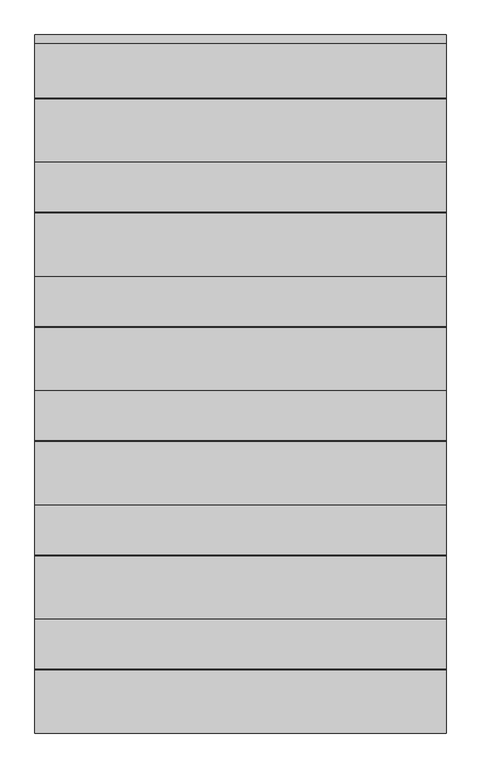
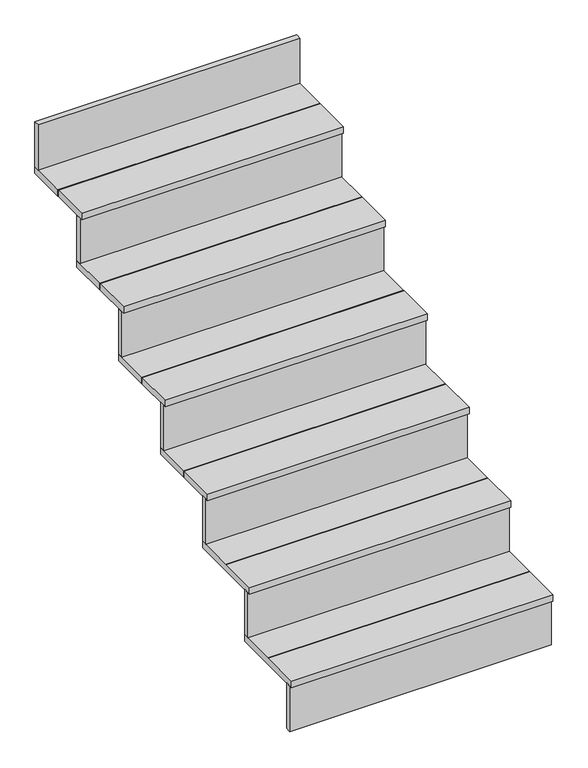
"""IFC4 building model written with IfcOpenShell, lengths in millimetres: stair flight geometry."""

from ifc_helpers import new_model, si_unit, frame, origin, origin_with_axes, place, context, project, spatial, polyline, outline, extrude, source, transform, mapped, element, save


def stair_flight_64412767(model_context):
    return source(origin(), model_context, "Body", "SweptSolid", [
        extrude(outline(polyline([(-21667.4414763, -10959.3570712), (-21667.4414763, -10978.4070712), (-22581.8414763, -10978.4070712), (-22581.8414763, -10959.3570712), (-21667.4414763, -10959.3570712)])), origin_with_axes(), (0.0, 0.0, 1.0), 167.8582813),
        extrude(outline(polyline([(-10848.2320712, 167.8582812), (-10987.9320712, 167.8582812), (-10987.9320712, 191.77), (-10848.2320712, 191.77), (-10848.2320712, 180.0157279), (-10845.0570712, 180.0157279), (-10845.0570712, 191.77), (-10705.3570712, 191.77), (-10705.3570712, 167.8582812), (-10845.0570712, 167.8582812), (-10845.0570712, 179.6125533), (-10848.2320712, 179.6125533), (-10848.2320712, 167.8582812)])), frame((-22581.8414763, 0.0, 0.0), z_axis=(1.0, 0.0, 0.0), x_axis=(0.0, 1.0, 0.0)), (0.0, 0.0, 1.0), 914.4),
        extrude(outline(polyline([(-21667.4414763, -10705.3570712), (-21667.4414763, -10724.4070712), (-22581.8414763, -10724.4070712), (-22581.8414763, -10705.3570712), (-21667.4414763, -10705.3570712)])), frame((0.0, 0.0, 191.77), z_axis=(0.0, 0.0, 1.0), x_axis=(1.0, 0.0, 0.0)), (0.0, 0.0, 1.0), 167.8582813),
        extrude(outline(polyline([(-10594.2320712, 359.6282812), (-10733.9320712, 359.6282812), (-10733.9320712, 383.54), (-10594.2320712, 383.54), (-10594.2320712, 371.7857279), (-10591.0570712, 371.7857279), (-10591.0570712, 383.54), (-10451.3570712, 383.54), (-10451.3570712, 359.6282812), (-10591.0570712, 359.6282812), (-10591.0570712, 371.3825533), (-10594.2320712, 371.3825533), (-10594.2320712, 359.6282812)])), frame((-22581.8414763, 0.0, 0.0), z_axis=(1.0, 0.0, 0.0), x_axis=(0.0, 1.0, 0.0)), (0.0, 0.0, 1.0), 914.4),
        extrude(outline(polyline([(-21667.4414763, -10451.3570712), (-21667.4414763, -10470.4070712), (-22581.8414763, -10470.4070712), (-22581.8414763, -10451.3570712), (-21667.4414763, -10451.3570712)])), frame((0.0, 0.0, 383.54), z_axis=(0.0, 0.0, 1.0), x_axis=(1.0, 0.0, 0.0)), (0.0, 0.0, 1.0), 167.8582813),
        extrude(outline(polyline([(-10340.2320712, 551.3982812), (-10479.9320712, 551.3982812), (-10479.9320712, 575.31), (-10340.2320712, 575.31), (-10340.2320712, 563.5557279), (-10337.0570712, 563.5557279), (-10337.0570712, 575.31), (-10197.3570712, 575.31), (-10197.3570712, 551.3982812), (-10337.0570712, 551.3982812), (-10337.0570712, 563.1525533), (-10340.2320712, 563.1525533), (-10340.2320712, 551.3982812)])), frame((-22581.8414763, 0.0, 0.0), z_axis=(1.0, 0.0, 0.0), x_axis=(0.0, 1.0, 0.0)), (0.0, 0.0, 1.0), 914.4),
        extrude(outline(polyline([(-21667.4414763, -10197.3570712), (-21667.4414763, -10216.4070712), (-22581.8414763, -10216.4070712), (-22581.8414763, -10197.3570712), (-21667.4414763, -10197.3570712)])), frame((0.0, 0.0, 575.31), z_axis=(0.0, 0.0, 1.0), x_axis=(1.0, 0.0, 0.0)), (0.0, 0.0, 1.0), 167.8582813),
        extrude(outline(polyline([(-10086.2320712, 743.1682812), (-10225.9320712, 743.1682812), (-10225.9320712, 767.08), (-10086.2320712, 767.08), (-10086.2320712, 755.3257279), (-10083.0570712, 755.3257279), (-10083.0570712, 767.08), (-9943.3570712, 767.08), (-9943.3570712, 743.1682812), (-10083.0570712, 743.1682812), (-10083.0570712, 754.9225533), (-10086.2320712, 754.9225533), (-10086.2320712, 743.1682812)])), frame((-22581.8414763, 0.0, 0.0), z_axis=(1.0, 0.0, 0.0), x_axis=(0.0, 1.0, 0.0)), (0.0, 0.0, 1.0), 914.4),
        extrude(outline(polyline([(-21667.4414763, -9943.3570712), (-21667.4414763, -9962.4070712), (-22581.8414763, -9962.4070712), (-22581.8414763, -9943.3570712), (-21667.4414763, -9943.3570712)])), frame((0.0, 0.0, 767.08), z_axis=(0.0, 0.0, 1.0), x_axis=(1.0, 0.0, 0.0)), (0.0, 0.0, 1.0), 167.8582813),
        extrude(outline(polyline([(-9832.2320712, 934.9382812), (-9971.9320712, 934.9382812), (-9971.9320712, 958.85), (-9832.2320712, 958.85), (-9832.2320712, 947.0957279), (-9829.0570712, 947.0957279), (-9829.0570712, 958.85), (-9689.3570712, 958.85), (-9689.3570712, 934.9382812), (-9829.0570712, 934.9382812), (-9829.0570712, 946.6925533), (-9832.2320712, 946.6925533), (-9832.2320712, 934.9382812)])), frame((-22581.8414763, 0.0, 0.0), z_axis=(1.0, 0.0, 0.0), x_axis=(0.0, 1.0, 0.0)), (0.0, 0.0, 1.0), 914.4),
        extrude(outline(polyline([(-21667.4414763, -9435.3570712), (-21667.4414763, -9454.4070712), (-22581.8414763, -9454.4070712), (-22581.8414763, -9435.3570712), (-21667.4414763, -9435.3570712)])), frame((0.0, 0.0, 1150.62), z_axis=(0.0, 0.0, 1.0), x_axis=(1.0, 0.0, 0.0)), (0.0, 0.0, 1.0), 167.8582812),
        extrude(outline(polyline([(-21667.4414763, -9689.3570712), (-21667.4414763, -9708.4070712), (-22581.8414763, -9708.4070712), (-22581.8414763, -9689.3570712), (-21667.4414763, -9689.3570712)])), frame((0.0, 0.0, 958.85), z_axis=(0.0, 0.0, 1.0), x_axis=(1.0, 0.0, 0.0)), (0.0, 0.0, 1.0), 167.8582813),
        extrude(outline(polyline([(-9578.2320712, 1126.7082813), (-9717.9320712, 1126.7082813), (-9717.9320712, 1150.62), (-9578.2320712, 1150.62), (-9578.2320712, 1138.8657279), (-9575.0570712, 1138.8657279), (-9575.0570712, 1150.62), (-9435.3570712, 1150.62), (-9435.3570712, 1126.7082812), (-9575.0570712, 1126.7082812), (-9575.0570712, 1138.4625533), (-9578.2320712, 1138.4625533), (-9578.2320712, 1126.7082813)])), frame((-22581.8414763, 0.0, 0.0), z_axis=(1.0, 0.0, 0.0), x_axis=(0.0, 1.0, 0.0)), (0.0, 0.0, 1.0), 914.4),
    ])


if __name__ == "__main__":
    model = new_model("IFC4")
    model_context = context("Model", 3, world=origin())
    ifc_project = project(units=[si_unit("LENGTHUNIT", "METRE", prefix="MILLI")], contexts=[model_context])
    site = spatial("IfcSite", under=ifc_project)
    building = spatial("IfcBuilding", under=site)
    placement = place(None, origin())
    stair_flight_shape = stair_flight_64412767(model_context)
    element("IfcStairFlight", 1, at=placement, inside=building, context=model_context, shape_type="MappedRepresentation", body=[
        mapped(stair_flight_shape, transform((0.0, 0.0, 0.0), x_axis=(1.0, 0.0, 0.0), y_axis=(0.0, 1.0, 0.0), z_axis=(0.0, 0.0, 1.0))),
    ])
    save(model, "model.ifc")

# Revit data of these elements
# Element 1 (IfcStairFlight)
#   Materials on its faces: "DEFAULT DOOR"
# Materials
#   "DEFAULT DOOR": class "Generic", colour RGB 216 216 216, transparency 0, Cost = 0
